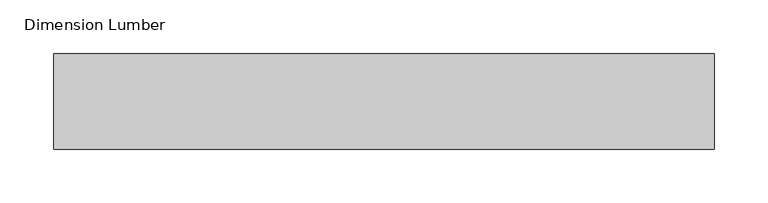
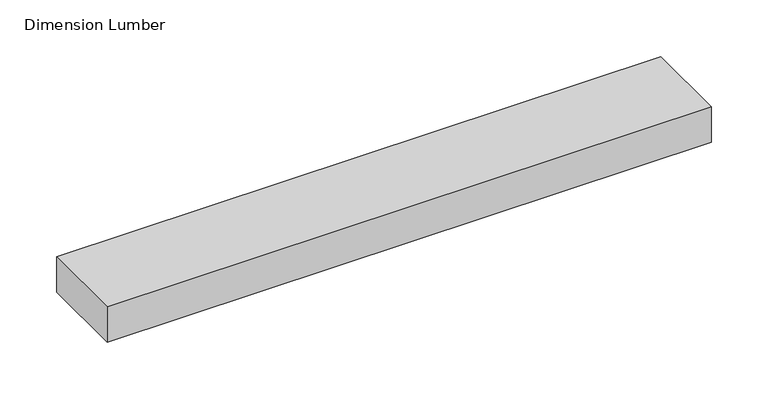
"""IFC4 building model written with IfcOpenShell, lengths in millimetres: beam geometry, Dimension Lumber : Top Supporting Lumbers."""

from ifc_helpers import new_model, si_unit, frame, origin, place, context, project, spatial, polyline, outline, extrude, source, transform, mapped, element, save


def dimension_lumber_4fd1e5d7(model_context):
    return source(origin(), model_context, "Body", "SweptSolid", [
        extrude(outline(polyline([(285.5562925, 44.45), (285.5562925, -44.45), (-330.0062925, -44.45), (-330.0062925, 44.45), (285.5562925, 44.45)])), frame((0.0, 0.0, -19.05), z_axis=(0.0, 0.0, 1.0), x_axis=(1.0, 0.0, 0.0)), (0.0, 0.0, 1.0), 38.1),
    ])


if __name__ == "__main__":
    model = new_model("IFC4")
    model_context = context("Model", 3, world=origin())
    ifc_project = project(units=[si_unit("LENGTHUNIT", "METRE", prefix="MILLI")], contexts=[model_context])
    site = spatial("IfcSite", under=ifc_project)
    building = spatial("IfcBuilding", under=site)
    placement = place(None, origin())
    dimension_lumber_shape = dimension_lumber_4fd1e5d7(model_context)
    element("IfcBeam", 1, ObjectType="Dimension Lumber : Top Supporting Lumbers", at=placement, inside=building, context=model_context, shape_type="MappedRepresentation", body=[
        mapped(dimension_lumber_shape, transform((0.0, 0.0, 0.0), x_axis=(1.0, 0.0, 0.0), y_axis=(0.0, 1.0, 0.0), z_axis=(0.0, 0.0, 1.0))),
    ])
    save(model, "model.ifc")

# Revit data of these elements
# Type "Dimension Lumber : Top Supporting Lumbers"
#   Assembly Code = "B10"
#   A = 0.0364583 SF
#   Length [instance default] = 5' - 0"
#   b = 0' - 3 1/2"
#   d = 0' - 1 1/2"
#   Structural Material [instance default] = Softwood, Lumber
# Element 1 (IfcBeam, "Dimension Lumber : Top Supporting Lumbers")
#   Structural Material = Douglas Fir #2
#   Materials on its faces: "Douglas Fir #2"
# Materials
#   "Softwood, Lumber": class "Wood", colour RGB 223 192 134, transparency 0, Description = "Pinus Echinata", Cost = 0
#   "Douglas Fir #2": class "Wood", colour RGB 223 192 134, transparency 0, Description = "Pinus Echinata", Cost = 0
